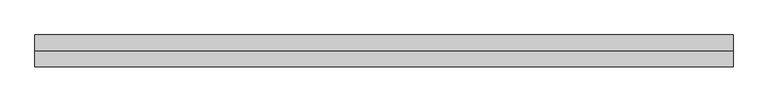
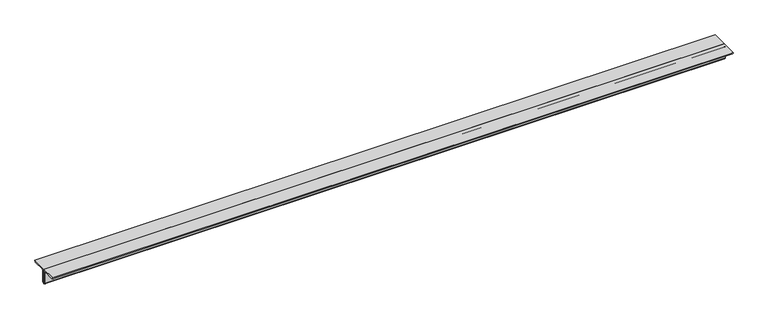
"""IFC4 building model written with IfcOpenShell, lengths in millimetres: member geometry, Steel Framing_2Ls_KS : H_SB_AR_S02_2Ls-100x100x10_VBR1."""

import ifcopenshell
import ifcopenshell.guid

model = None  # the IFC model being written
_history = None  # IfcOwnerHistory: only IFC2X3 demands one
_inside = {}  # id of a spatial element -> (the spatial element, [elements in it])
_under = {}  # id of a project, library or spatial element -> (it, [spatial elements below it])
_declared = {}  # id of a project -> (the project, [libraries it declares])
_typed = {}  # id of a type object -> (the type object, [elements of that type])
_made_of = {}  # id of a material, layer set ... -> (it, [elements and type objects made of it])


def new_model(schema):
    """Start an empty IFC model of exactly this schema.

    Asked for "IFC4X3", IfcOpenShell would pick the latest addendum, in which some entities
    have other attributes; the version numbers below select the first issue.
    IFC2X3 requires an IfcOwnerHistory on every rooted entity: one is made here for all.
    """
    global model, _history
    if schema == "IFC4X3":
        model = ifcopenshell.file(schema_version=(4, 3, 0, 0))
    else:
        model = ifcopenshell.file(schema=schema)
    _inside.clear()
    _under.clear()
    _declared.clear()
    _typed.clear()
    _made_of.clear()
    _history = None
    if model.schema == "IFC2X3":
        org = make("IfcOrganization", Name="unknown")
        user = make(
            "IfcPersonAndOrganization",
            ThePerson=make("IfcPerson", FamilyName="unknown"),
            TheOrganization=org,
        )
        app = make(
            "IfcApplication",
            ApplicationDeveloper=org,
            Version="unknown",
            ApplicationFullName="unknown",
            ApplicationIdentifier="unknown",
        )
        _history = make(
            "IfcOwnerHistory",
            OwningUser=user,
            OwningApplication=app,
            ChangeAction="ADDED",
            CreationDate=0,
        )
    return model


def make(cls, **values):
    """One entity of the class cls with the attributes given. An attribute that is None is left unset."""
    return model.create_entity(
        cls, **{name: value for name, value in values.items() if value is not None}
    )


def rooted(cls, **values):
    """An entity with a GlobalId (a new one), such as an element, a storey or a relation."""
    return make(cls, GlobalId=ifcopenshell.guid.new(), OwnerHistory=_history, **values)


def si_unit(unit_type, name, prefix=None):
    """IfcSIUnit, for example si_unit("LENGTHUNIT", "METRE", prefix="MILLI")."""
    return make("IfcSIUnit", UnitType=unit_type, Prefix=prefix, Name=name)


def assignment(units):
    """IfcUnitAssignment: the units of a project."""
    return None if units is None else make("IfcUnitAssignment", Units=units)


def point(xyz):
    """IfcCartesianPoint."""
    return None if xyz is None else make("IfcCartesianPoint", Coordinates=xyz)


def direction(xyz):
    """IfcDirection."""
    return None if xyz is None else make("IfcDirection", DirectionRatios=xyz)


def frame(location, z_axis=None, x_axis=None):
    """IfcAxis2Placement3D, a coordinate frame: its origin and axes. An axis left out is left unset."""
    return make(
        "IfcAxis2Placement3D",
        Location=point(location),
        Axis=direction(z_axis),
        RefDirection=direction(x_axis),
    )


def frame_2d(location, x_axis=None):
    """IfcAxis2Placement2D, a coordinate frame in the plane: its origin and x axis."""
    return make(
        "IfcAxis2Placement2D", Location=point(location), RefDirection=direction(x_axis)
    )


def origin():
    """The frame at (0, 0, 0) with its axes left unset."""
    return frame((0.0, 0.0, 0.0))


def place(relative_to, where):
    """IfcLocalPlacement: puts the frame where relative to a parent placement (None: the world)."""
    return make(
        "IfcLocalPlacement", PlacementRelTo=relative_to, RelativePlacement=where
    )


def context(
    kind, dimensions, precision=None, world=None, true_north=None, identifier=None
):
    """IfcGeometricRepresentationContext, for example the 3D "Model" context."""
    return make(
        "IfcGeometricRepresentationContext",
        ContextIdentifier=identifier,
        ContextType=kind,
        CoordinateSpaceDimension=dimensions,
        Precision=precision,
        WorldCoordinateSystem=world,
        TrueNorth=true_north,
    )


def project(units=None, contexts=None):
    """IfcProject with its units and contexts."""
    return rooted(
        "IfcProject",
        Name="project",
        RepresentationContexts=contexts,
        UnitsInContext=assignment(units),
    )


def spatial(cls, under=None, at=None, **own):
    """A site, building, storey or space (cls), placed at a placement, below another one or the project."""
    s = rooted(cls, ObjectPlacement=at, **own)
    if under is not None:
        _under.setdefault(under.id(), (under, []))[1].append(s)
    return s


def polyline(points):
    """IfcPolyline through the points."""
    return make("IfcPolyline", Points=[point(p) for p in points])


def circle_curve(where, radius):
    """IfcCircle in the frame where."""
    return make("IfcCircle", Position=where, Radius=radius)


def trimmed(basis, trim1, trim2, sense, master):
    """IfcTrimmedCurve: the piece of a basis curve between two trims."""
    return make(
        "IfcTrimmedCurve",
        BasisCurve=basis,
        Trim1=trim1,
        Trim2=trim2,
        SenseAgreement=sense,
        MasterRepresentation=master,
    )


def segment(curve, same_sense, transition):
    """IfcCompositeCurveSegment."""
    return make(
        "IfcCompositeCurveSegment",
        Transition=transition,
        SameSense=same_sense,
        ParentCurve=curve,
    )


def composite_curve(segments, self_intersect=None):
    """IfcCompositeCurve: segments joined end to end."""
    return make("IfcCompositeCurve", Segments=segments, SelfIntersect=self_intersect)


def outline(outer, holes=None, kind="AREA"):
    """IfcArbitraryClosedProfileDef: a profile drawn as a closed curve; with holes, ...WithVoids."""
    if holes is None:
        return make("IfcArbitraryClosedProfileDef", ProfileType=kind, OuterCurve=outer)
    return make(
        "IfcArbitraryProfileDefWithVoids",
        ProfileType=kind,
        OuterCurve=outer,
        InnerCurves=holes,
    )


def extrude(swept, where, along, depth):
    """IfcExtrudedAreaSolid: the profile swept, set in the frame where, extruded along a direction by depth."""
    return make(
        "IfcExtrudedAreaSolid",
        SweptArea=swept,
        Position=where,
        ExtrudedDirection=direction(along),
        Depth=depth,
    )


def shape(context_of_items, identifier, shape_type, items):
    """IfcShapeRepresentation: the items that make up one representation, for example the "Body"."""
    return make(
        "IfcShapeRepresentation",
        ContextOfItems=context_of_items,
        RepresentationIdentifier=identifier,
        RepresentationType=shape_type,
        Items=items,
    )


def source(mapping_origin, context_of_items, identifier, shape_type, items):
    """IfcRepresentationMap: a shape defined once, which mapped items show again and again."""
    return make(
        "IfcRepresentationMap",
        MappingOrigin=mapping_origin,
        MappedRepresentation=shape(context_of_items, identifier, shape_type, items),
    )


def transform(
    local_origin,
    x_axis=None,
    y_axis=None,
    z_axis=None,
    scale=None,
    scale2=None,
    scale3=None,
    uniform=True,
):
    """IfcCartesianTransformationOperator3D, or its non-uniform kind. x_axis, y_axis, z_axis: its Axis1, 2, 3."""
    if uniform:
        return make(
            "IfcCartesianTransformationOperator3D",
            Axis1=direction(x_axis),
            Axis2=direction(y_axis),
            LocalOrigin=point(local_origin),
            Scale=scale,
            Axis3=direction(z_axis),
        )
    return make(
        "IfcCartesianTransformationOperator3DnonUniform",
        Axis1=direction(x_axis),
        Axis2=direction(y_axis),
        LocalOrigin=point(local_origin),
        Scale=scale,
        Axis3=direction(z_axis),
        Scale2=scale2,
        Scale3=scale3,
    )


def mapped(mapping_source, mapping_target):
    """IfcMappedItem: shows the shape of a source again, moved by a transform."""
    return make(
        "IfcMappedItem", MappingSource=mapping_source, MappingTarget=mapping_target
    )


def made_of(thing, what):
    """Note that an element or type object is made of a material, layer set ...; save() writes the relation."""
    if what is not None:
        _made_of.setdefault(what.id(), (what, []))[1].append(thing)
    return thing


def element(
    cls,
    number,
    at=None,
    inside=None,
    cuts=None,
    type_object=None,
    material=None,
    context=None,
    identifier="Body",
    shape_type=None,
    held_by="IfcProductDefinitionShape",
    body=None,
    shapes=None,
    **own,
):
    """One element of the class cls, such as IfcWall. Its Tag is "e" and its number.

    at: its placement. inside: the storey or other place that contains it. cuts: it is an
    opening in that element (IfcRelVoidsElement). A single representation is given by context,
    identifier, shape_type and body (its items); several are given by shapes. held_by: the class
    of the entity that holds the representations. save() writes the other relations.
    """
    e = rooted(cls, Tag="e%d" % number, ObjectPlacement=at, **own)
    if body is not None:
        shapes = [shape(context, identifier, shape_type, body)]
    if shapes is not None:
        e.Representation = make(held_by, Representations=shapes)
    if inside is not None:
        _inside.setdefault(inside.id(), (inside, []))[1].append(e)
    if cuts is not None:
        rooted(
            "IfcRelVoidsElement", RelatingBuildingElement=cuts, RelatedOpeningElement=e
        )
    if type_object is not None:
        _typed.setdefault(type_object.id(), (type_object, []))[1].append(e)
    return made_of(e, material)


def aggregate(whole, parts):
    """IfcRelAggregates: a whole, such as a stair, and the parts it consists of."""
    return rooted("IfcRelAggregates", RelatingObject=whole, RelatedObjects=parts)


def save(model, path):
    """Write the relations noted so far, then the file.

    IfcRelAggregates (storeys below a building ...), IfcRelContainedInSpatialStructure (elements
    in a storey), IfcRelDefinesByType, IfcRelAssociatesMaterial and IfcRelDeclares: one each for
    every whole, place, type object, material and project.
    """
    for whole, parts in _under.values():
        aggregate(whole, parts)
    for where, things in _inside.values():
        rooted(
            "IfcRelContainedInSpatialStructure",
            RelatedElements=things,
            RelatingStructure=where,
        )
    for kind, things in _typed.values():
        rooted("IfcRelDefinesByType", RelatedObjects=things, RelatingType=kind)
    for what, things in _made_of.values():
        rooted("IfcRelAssociatesMaterial", RelatedObjects=things, RelatingMaterial=what)
    for by, libraries in _declared.values():
        rooted("IfcRelDeclares", RelatingContext=by, RelatedDefinitions=libraries)
    model.write(path)


def member_0cbf2c2f(model_context):
    return source(origin(), model_context, "Body", "SweptSolid", [
        extrude(outline(composite_curve([segment(polyline([(0.0, 28.2), (100.0, 28.2)]), True, "CONTINUOUS"), segment(trimmed(circle_curve(frame_2d((90.0, 28.2)), 10.0), [point((100.0, 28.2))], [point((90.0, 18.2))], False, "CARTESIAN"), True, "CONTINUOUS"), segment(polyline([(90.0, 18.2), (20.0, 18.2)]), True, "CONTINUOUS"), segment(trimmed(circle_curve(frame_2d((20.0, 8.2)), 10.0), [point((20.0, 18.2))], [point((10.0, 8.2))], True, "CARTESIAN"), True, "CONTINUOUS"), segment(polyline([(10.0, 8.2), (10.0, -61.8)]), True, "CONTINUOUS"), segment(trimmed(circle_curve(frame_2d((0.0, -61.8)), 10.0), [point((10.0, -61.8))], [point((0.0, -71.8))], False, "CARTESIAN"), True, "CONTINUOUS"), segment(polyline([(0.0, -71.8), (0.0, 28.2)]), True, "CONTINUOUS")], self_intersect=False)), frame((-2041.6751257, 0.0, 0.0), z_axis=(1.0, 0.0, 0.0), x_axis=(0.0, 1.0, 0.0)), (0.0, 0.0, 1.0), 4392.2791792),
        extrude(outline(composite_curve([segment(polyline([(0.0, 28.2), (0.0, -71.8)]), True, "CONTINUOUS"), segment(trimmed(circle_curve(frame_2d((0.0, -61.8)), 10.0), [point((0.0, -71.8))], [point((-10.0, -61.8))], False, "CARTESIAN"), True, "CONTINUOUS"), segment(polyline([(-10.0, -61.8), (-10.0, 8.2)]), True, "CONTINUOUS"), segment(trimmed(circle_curve(frame_2d((-20.0, 8.2)), 10.0), [point((-10.0, 8.2))], [point((-20.0, 18.2))], True, "CARTESIAN"), True, "CONTINUOUS"), segment(polyline([(-20.0, 18.2), (-90.0, 18.2)]), True, "CONTINUOUS"), segment(trimmed(circle_curve(frame_2d((-90.0, 28.2)), 10.0), [point((-90.0, 18.2))], [point((-100.0, 28.2))], False, "CARTESIAN"), True, "CONTINUOUS"), segment(polyline([(-100.0, 28.2), (0.0, 28.2)]), True, "CONTINUOUS")], self_intersect=False)), frame((-2041.6751257, 0.0, 0.0), z_axis=(1.0, 0.0, 0.0), x_axis=(0.0, 1.0, 0.0)), (0.0, 0.0, 1.0), 4392.2791792),
    ])


if __name__ == "__main__":
    model = new_model("IFC4")
    model_context = context("Model", 3, world=origin())
    ifc_project = project(units=[si_unit("LENGTHUNIT", "METRE", prefix="MILLI")], contexts=[model_context])
    site = spatial("IfcSite", under=ifc_project)
    building = spatial("IfcBuilding", under=site)
    placement = place(None, origin())
    member_shape = member_0cbf2c2f(model_context)
    element("IfcMember", 1, ObjectType="Steel Framing_2Ls_KS : H_SB_AR_S02_2Ls-100x100x10_VBR1", at=placement, inside=building, context=model_context, shape_type="MappedRepresentation", body=[
        mapped(member_shape, transform((0.0, 0.0, 0.0), x_axis=(1.0, 0.0, 0.0), y_axis=(0.0, 1.0, 0.0), z_axis=(0.0, 0.0, 1.0))),
    ])
    save(model, "model.ifc")

# Revit data of these elements
# Type "Steel Framing_2Ls_KS : H_SB_AR_S02_2Ls-100x100x10_VBR1"
#   Type Comments = "MAIN"
#   Type Mark = "VBR1"
#   H_SectionID = "2Ls-100x100x10"
#   Assembly Code = "B10"
#   Legs = "LLBB"
#   H_Ratio for Additional Steel Plate = 0.2
#   W = 0
#   Perimeter = 0.80 m²/m
#   Nominal Weight = 29.80 kgf/m
#   Length [instance default] = 1524 mm
#   Space = 0 mm
#   b = 100 mm
#   d = 100 mm
#   t = 10 mm
#   y = 28.2 mm
#   A = 0.0038 m²
#   Structural Material [instance default] = Steel, 45-345
# Element 1 (IfcMember, "Steel Framing_2Ls_KS : H_SB_AR_S02_2Ls-100x100x10_VBR1")
#   Materials on its faces: "Steel, 45-345"
# Materials
#   "Steel, 45-345": class "Metal", colour RGB 189 187 185, transparency 0, Description = "Steel 345 MPa", Cost = 0
